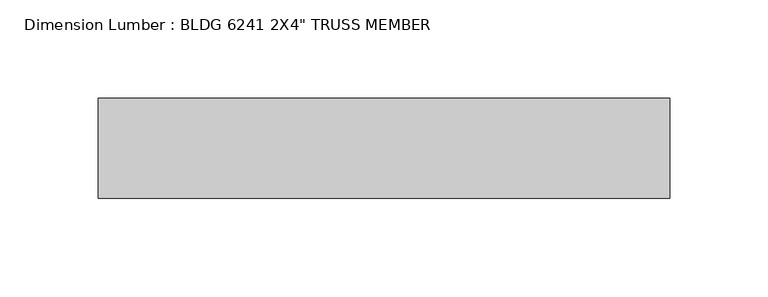
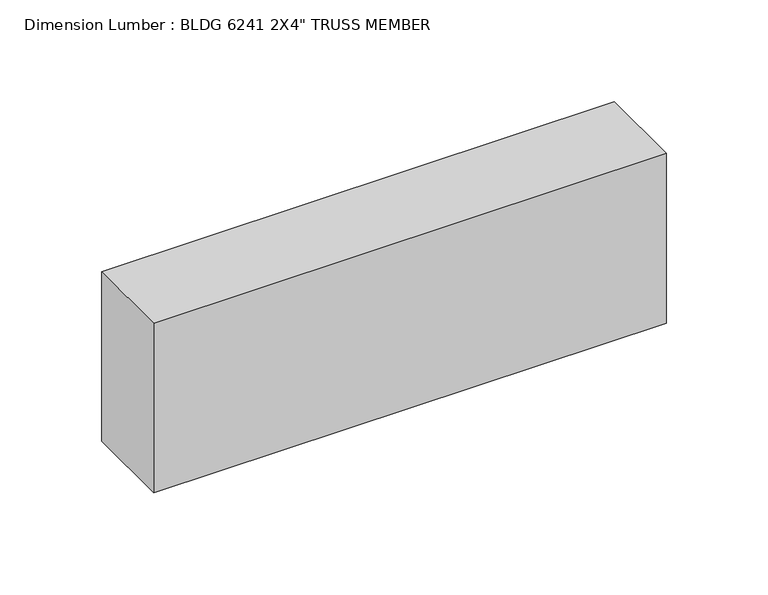
"""IFC4 building model written with IfcOpenShell, lengths in millimetres: beam geometry."""

from ifc_helpers import new_model, si_unit, frame, origin, place, context, project, spatial, polyline, outline, extrude, source, transform, mapped, element, save


def beam_87710fdd(model_context):
    return source(origin(), model_context, "Body", "SweptSolid", [
        extrude(outline(polyline([(147.1272806, 25.4), (147.1272806, -25.4), (-142.875, -25.4), (-142.875, 25.4), (147.1272806, 25.4)])), frame((0.0, 0.0, -50.8), z_axis=(0.0, 0.0, 1.0), x_axis=(1.0, 0.0, 0.0)), (0.0, 0.0, 1.0), 101.6),
    ])


if __name__ == "__main__":
    model = new_model("IFC4")
    model_context = context("Model", 3, world=origin())
    ifc_project = project(units=[si_unit("LENGTHUNIT", "METRE", prefix="MILLI")], contexts=[model_context])
    site = spatial("IfcSite", under=ifc_project)
    building = spatial("IfcBuilding", under=site)
    placement = place(None, origin())
    beam_shape = beam_87710fdd(model_context)
    element("IfcBeam", 1, ObjectType="Dimension Lumber : BLDG 6241 2X4\" TRUSS MEMBER", at=placement, inside=building, context=model_context, shape_type="MappedRepresentation", body=[
        mapped(beam_shape, transform((0.0, 0.0, 0.0), x_axis=(1.0, 0.0, 0.0), y_axis=(0.0, 1.0, 0.0), z_axis=(0.0, 0.0, 1.0))),
    ])
    save(model, "model.ifc")

# Revit data of these elements
# Type "Dimension Lumber : BLDG 6241 2X4\" TRUSS MEMBER"
#   Assembly Code = "B10"
#   A = 0.273472 SF
#   Length [instance default] = 5' - 0"
#   b = 0' - 2"
#   d = 0' - 4"
#   Structural Material [instance default] = Softwood, Lumber
# Element 1 (IfcBeam, "Dimension Lumber : BLDG 6241 2X4\" TRUSS MEMBER")
#   Materials on its faces: "Softwood, Lumber"
# Materials
#   "Softwood, Lumber": class "Wood", colour RGB 223 192 134, transparency 0, Description = "Pinus Echinata", Cost = 0
